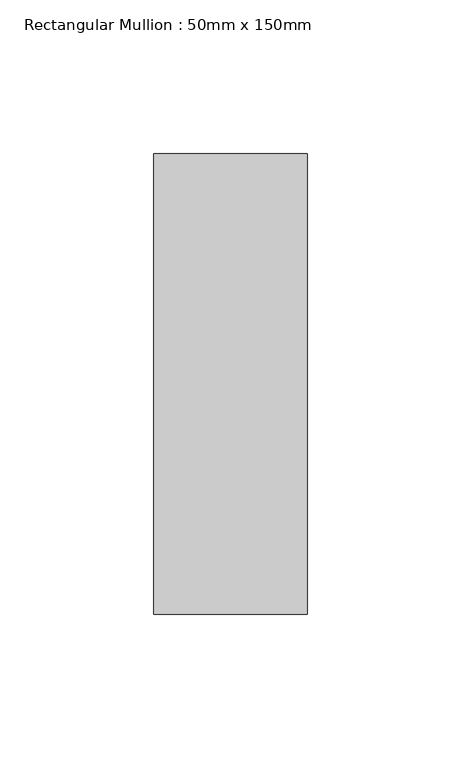
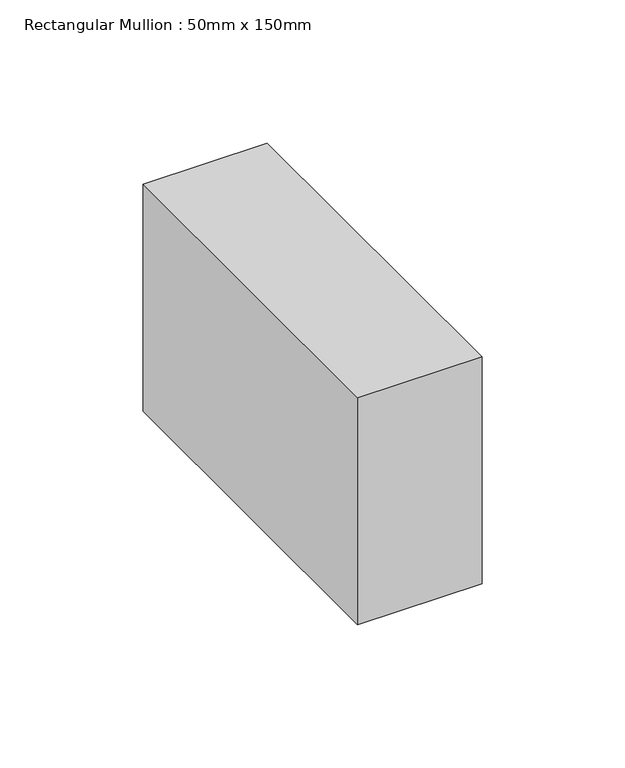
"""IFC4 building model written with IfcOpenShell, lengths in millimetres: member geometry, Rectangular Mullion : 50mm x 150mm."""

from ifc_helpers import new_model, si_unit, frame, origin, place, context, project, spatial, polyline, outline, extrude, source, transform, mapped, element, save


def rectangular_mullion_50mm_x_150mm_80e47556(model_context):
    return source(origin(), model_context, "Body", "SweptSolid", [
        extrude(outline(polyline([(0.0, 75.0), (0.0, -75.0), (-50.0, -75.0), (-50.0, 75.0), (0.0, 75.0)])), frame((0.0, 0.0, -96.8181816), z_axis=(0.0, 0.0, 1.0), x_axis=(1.0, 0.0, 0.0)), (0.0, 0.0, 1.0), 96.8181816),
    ])


if __name__ == "__main__":
    model = new_model("IFC4")
    model_context = context("Model", 3, world=origin())
    ifc_project = project(units=[si_unit("LENGTHUNIT", "METRE", prefix="MILLI")], contexts=[model_context])
    site = spatial("IfcSite", under=ifc_project)
    building = spatial("IfcBuilding", under=site)
    placement = place(None, origin())
    rectangular_mullion_50mm_x_150mm_shape = rectangular_mullion_50mm_x_150mm_80e47556(model_context)
    element("IfcMember", 1, ObjectType="Rectangular Mullion : 50mm x 150mm", at=placement, inside=building, context=model_context, shape_type="MappedRepresentation", body=[
        mapped(rectangular_mullion_50mm_x_150mm_shape, transform((0.0, 0.0, 0.0), x_axis=(1.0, 0.0, 0.0), y_axis=(0.0, 1.0, 0.0), z_axis=(0.0, 0.0, 1.0))),
    ])
    save(model, "model.ifc")

# Revit data of these elements
# Type "Rectangular Mullion : 50mm x 150mm"
#   built-in parameter 1007304 = 0.492126 (stored number, unit not read)
#   built-in parameter 1007301 = 0.082021 (stored number, unit not read)
#   built-in parameter 1007300 = 0.082021 (stored number, unit not read)
# Element 1 (IfcMember, "Rectangular Mullion : 50mm x 150mm")
#   Materials on its faces: "Aluminum"
# Materials
#   "Aluminum": class "Metal", colour RGB 244 244 244, transparency 0, Description = "Aluminum 6061", Cost = 0
